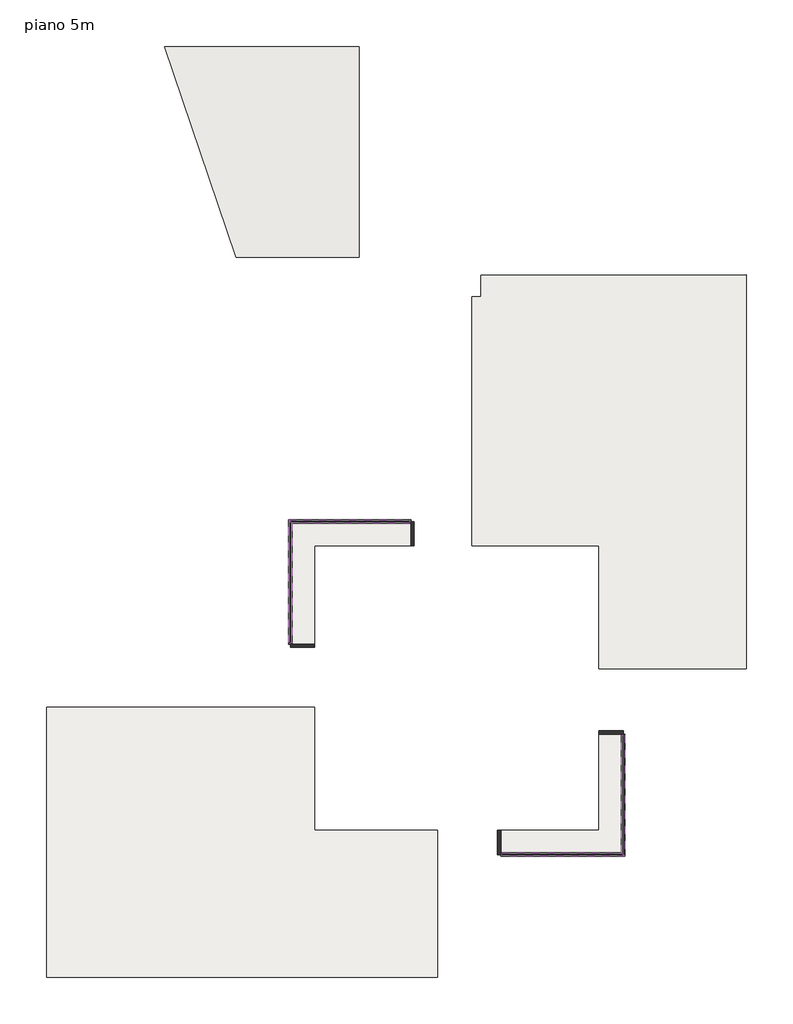
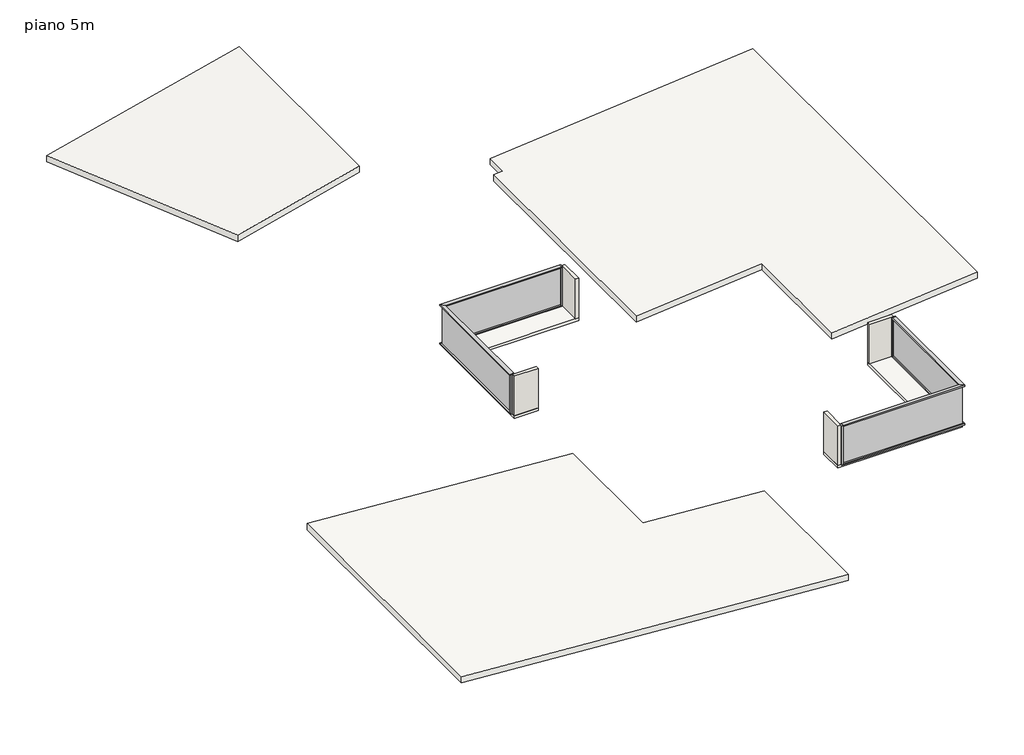
# One storey: 12 members, 4 plates, 4 walls, 3 roofs, 2 slabs.
"""IFC4 building model written with IfcOpenShell, lengths in millimetres."""

import ifcopenshell
import ifcopenshell.guid

model = None  # the IFC model being written
_history = None  # IfcOwnerHistory: only IFC2X3 demands one
_inside = {}  # id of a spatial element -> (the spatial element, [elements in it])
_under = {}  # id of a project, library or spatial element -> (it, [spatial elements below it])
_declared = {}  # id of a project -> (the project, [libraries it declares])
_typed = {}  # id of a type object -> (the type object, [elements of that type])
_made_of = {}  # id of a material, layer set ... -> (it, [elements and type objects made of it])


def new_model(schema):
    """Start an empty IFC model of exactly this schema.

    Asked for "IFC4X3", IfcOpenShell would pick the latest addendum, in which some entities
    have other attributes; the version numbers below select the first issue.
    IFC2X3 requires an IfcOwnerHistory on every rooted entity: one is made here for all.
    """
    global model, _history
    if schema == "IFC4X3":
        model = ifcopenshell.file(schema_version=(4, 3, 0, 0))
    else:
        model = ifcopenshell.file(schema=schema)
    _inside.clear()
    _under.clear()
    _declared.clear()
    _typed.clear()
    _made_of.clear()
    _history = None
    if model.schema == "IFC2X3":
        org = make("IfcOrganization", Name="unknown")
        user = make(
            "IfcPersonAndOrganization",
            ThePerson=make("IfcPerson", FamilyName="unknown"),
            TheOrganization=org,
        )
        app = make(
            "IfcApplication",
            ApplicationDeveloper=org,
            Version="unknown",
            ApplicationFullName="unknown",
            ApplicationIdentifier="unknown",
        )
        _history = make(
            "IfcOwnerHistory",
            OwningUser=user,
            OwningApplication=app,
            ChangeAction="ADDED",
            CreationDate=0,
        )
    return model


def make(cls, **values):
    """One entity of the class cls with the attributes given. An attribute that is None is left unset."""
    return model.create_entity(
        cls, **{name: value for name, value in values.items() if value is not None}
    )


def rooted(cls, **values):
    """An entity with a GlobalId (a new one), such as an element, a storey or a relation."""
    return make(cls, GlobalId=ifcopenshell.guid.new(), OwnerHistory=_history, **values)


def si_unit(unit_type, name, prefix=None):
    """IfcSIUnit, for example si_unit("LENGTHUNIT", "METRE", prefix="MILLI")."""
    return make("IfcSIUnit", UnitType=unit_type, Prefix=prefix, Name=name)


def assignment(units):
    """IfcUnitAssignment: the units of a project."""
    return None if units is None else make("IfcUnitAssignment", Units=units)


def point(xyz):
    """IfcCartesianPoint."""
    return None if xyz is None else make("IfcCartesianPoint", Coordinates=xyz)


def direction(xyz):
    """IfcDirection."""
    return None if xyz is None else make("IfcDirection", DirectionRatios=xyz)


def frame(location, z_axis=None, x_axis=None):
    """IfcAxis2Placement3D, a coordinate frame: its origin and axes. An axis left out is left unset."""
    return make(
        "IfcAxis2Placement3D",
        Location=point(location),
        Axis=direction(z_axis),
        RefDirection=direction(x_axis),
    )


def origin():
    """The frame at (0, 0, 0) with its axes left unset."""
    return frame((0.0, 0.0, 0.0))


def origin_with_axes():
    """The frame at (0, 0, 0) with the z axis (0, 0, 1) and the x axis (1, 0, 0) written out."""
    return frame((0.0, 0.0, 0.0), z_axis=(0.0, 0.0, 1.0), x_axis=(1.0, 0.0, 0.0))


def place(relative_to, where):
    """IfcLocalPlacement: puts the frame where relative to a parent placement (None: the world)."""
    return make(
        "IfcLocalPlacement", PlacementRelTo=relative_to, RelativePlacement=where
    )


def context(
    kind, dimensions, precision=None, world=None, true_north=None, identifier=None
):
    """IfcGeometricRepresentationContext, for example the 3D "Model" context."""
    return make(
        "IfcGeometricRepresentationContext",
        ContextIdentifier=identifier,
        ContextType=kind,
        CoordinateSpaceDimension=dimensions,
        Precision=precision,
        WorldCoordinateSystem=world,
        TrueNorth=true_north,
    )


def project(units=None, contexts=None):
    """IfcProject with its units and contexts."""
    return rooted(
        "IfcProject",
        Name="project",
        RepresentationContexts=contexts,
        UnitsInContext=assignment(units),
    )


def spatial(cls, under=None, at=None, **own):
    """A site, building, storey or space (cls), placed at a placement, below another one or the project."""
    s = rooted(cls, ObjectPlacement=at, **own)
    if under is not None:
        _under.setdefault(under.id(), (under, []))[1].append(s)
    return s


def polyline(points):
    """IfcPolyline through the points."""
    return make("IfcPolyline", Points=[point(p) for p in points])


def outline(outer, holes=None, kind="AREA"):
    """IfcArbitraryClosedProfileDef: a profile drawn as a closed curve; with holes, ...WithVoids."""
    if holes is None:
        return make("IfcArbitraryClosedProfileDef", ProfileType=kind, OuterCurve=outer)
    return make(
        "IfcArbitraryProfileDefWithVoids",
        ProfileType=kind,
        OuterCurve=outer,
        InnerCurves=holes,
    )


def extrude(swept, where, along, depth):
    """IfcExtrudedAreaSolid: the profile swept, set in the frame where, extruded along a direction by depth."""
    return make(
        "IfcExtrudedAreaSolid",
        SweptArea=swept,
        Position=where,
        ExtrudedDirection=direction(along),
        Depth=depth,
    )


def faces_of(points, faces, orient=None, outer=None):
    """IfcFace entities. A face is a list of loops; a loop is a list of indices into points, from 0.

    orient and outer hold one flag for each loop. By default every Orientation is true, the
    first loop of a face is its IfcFaceOuterBound and the others are IfcFaceBound.
    """
    made = []
    for i, loops in enumerate(faces):
        bounds = []
        for j, loop in enumerate(loops):
            is_outer = j == 0 if outer is None else outer[i][j]
            bounds.append(
                make(
                    "IfcFaceOuterBound" if is_outer else "IfcFaceBound",
                    Bound=make("IfcPolyLoop", Polygon=[points[k] for k in loop]),
                    Orientation=True if orient is None else orient[i][j],
                )
            )
        made.append(make("IfcFace", Bounds=bounds))
    return made


def faceted_brep(points, faces, orient=None, outer=None, voids=None):
    """IfcFacetedBrep: a solid bounded by flat faces; with voids (closed shells), ...WithVoids."""
    shared = [point(p) for p in points]
    hull = make("IfcClosedShell", CfsFaces=faces_of(shared, faces, orient, outer))
    if voids is None:
        return make("IfcFacetedBrep", Outer=hull)
    return make(
        "IfcFacetedBrepWithVoids",
        Outer=hull,
        Voids=[
            make(cls, CfsFaces=faces_of(shared, fs, o, b)) for cls, fs, o, b in voids
        ],
    )


def shape(context_of_items, identifier, shape_type, items):
    """IfcShapeRepresentation: the items that make up one representation, for example the "Body"."""
    return make(
        "IfcShapeRepresentation",
        ContextOfItems=context_of_items,
        RepresentationIdentifier=identifier,
        RepresentationType=shape_type,
        Items=items,
    )


def source(mapping_origin, context_of_items, identifier, shape_type, items):
    """IfcRepresentationMap: a shape defined once, which mapped items show again and again."""
    return make(
        "IfcRepresentationMap",
        MappingOrigin=mapping_origin,
        MappedRepresentation=shape(context_of_items, identifier, shape_type, items),
    )


def transform(
    local_origin,
    x_axis=None,
    y_axis=None,
    z_axis=None,
    scale=None,
    scale2=None,
    scale3=None,
    uniform=True,
):
    """IfcCartesianTransformationOperator3D, or its non-uniform kind. x_axis, y_axis, z_axis: its Axis1, 2, 3."""
    if uniform:
        return make(
            "IfcCartesianTransformationOperator3D",
            Axis1=direction(x_axis),
            Axis2=direction(y_axis),
            LocalOrigin=point(local_origin),
            Scale=scale,
            Axis3=direction(z_axis),
        )
    return make(
        "IfcCartesianTransformationOperator3DnonUniform",
        Axis1=direction(x_axis),
        Axis2=direction(y_axis),
        LocalOrigin=point(local_origin),
        Scale=scale,
        Axis3=direction(z_axis),
        Scale2=scale2,
        Scale3=scale3,
    )


def mapped(mapping_source, mapping_target):
    """IfcMappedItem: shows the shape of a source again, moved by a transform."""
    return make(
        "IfcMappedItem", MappingSource=mapping_source, MappingTarget=mapping_target
    )


def made_of(thing, what):
    """Note that an element or type object is made of a material, layer set ...; save() writes the relation."""
    if what is not None:
        _made_of.setdefault(what.id(), (what, []))[1].append(thing)
    return thing


def element(
    cls,
    number,
    at=None,
    inside=None,
    cuts=None,
    type_object=None,
    material=None,
    context=None,
    identifier="Body",
    shape_type=None,
    held_by="IfcProductDefinitionShape",
    body=None,
    shapes=None,
    **own,
):
    """One element of the class cls, such as IfcWall. Its Tag is "e" and its number.

    at: its placement. inside: the storey or other place that contains it. cuts: it is an
    opening in that element (IfcRelVoidsElement). A single representation is given by context,
    identifier, shape_type and body (its items); several are given by shapes. held_by: the class
    of the entity that holds the representations. save() writes the other relations.
    """
    e = rooted(cls, Tag="e%d" % number, ObjectPlacement=at, **own)
    if body is not None:
        shapes = [shape(context, identifier, shape_type, body)]
    if shapes is not None:
        e.Representation = make(held_by, Representations=shapes)
    if inside is not None:
        _inside.setdefault(inside.id(), (inside, []))[1].append(e)
    if cuts is not None:
        rooted(
            "IfcRelVoidsElement", RelatingBuildingElement=cuts, RelatedOpeningElement=e
        )
    if type_object is not None:
        _typed.setdefault(type_object.id(), (type_object, []))[1].append(e)
    return made_of(e, material)


def aggregate(whole, parts):
    """IfcRelAggregates: a whole, such as a stair, and the parts it consists of."""
    return rooted("IfcRelAggregates", RelatingObject=whole, RelatedObjects=parts)


def save(model, path):
    """Write the relations noted so far, then the file.

    IfcRelAggregates (storeys below a building ...), IfcRelContainedInSpatialStructure (elements
    in a storey), IfcRelDefinesByType, IfcRelAssociatesMaterial and IfcRelDeclares: one each for
    every whole, place, type object, material and project.
    """
    for whole, parts in _under.values():
        aggregate(whole, parts)
    for where, things in _inside.values():
        rooted(
            "IfcRelContainedInSpatialStructure",
            RelatedElements=things,
            RelatingStructure=where,
        )
    for kind, things in _typed.values():
        rooted("IfcRelDefinesByType", RelatedObjects=things, RelatingType=kind)
    for what, things in _made_of.values():
        rooted("IfcRelAssociatesMaterial", RelatedObjects=things, RelatingMaterial=what)
    for by, libraries in _declared.values():
        rooted("IfcRelDeclares", RelatingContext=by, RelatedDefinitions=libraries)
    model.write(path)


def montante_rettangolare_montante_rettangolare_b878ced1(model_context):
    return source(origin(), model_context, "Body", "SweptSolid", [
        extrude(outline(polyline([(0.0, 75.0), (0.0, -75.0), (-50.0, -75.0), (-50.0, 75.0), (0.0, 75.0)])), frame((0.0, 0.0, -1745.0), z_axis=(0.0, 0.0, 1.0), x_axis=(1.0, 0.0, 0.0)), (0.0, 0.0, 1.0), 1745.0),
    ])


def montante_rettangolare_montante_rettangolare_f37d3d93(model_context):
    return source(origin(), model_context, "Body", "SweptSolid", [
        extrude(outline(polyline([(-75.0, -75.0), (75.0, 75.0), (75.0, -4920.0), (-75.0, -4920.0), (-75.0, -75.0)])), frame((-50.0, 0.0, 0.0), z_axis=(1.0, 0.0, 0.0), x_axis=(0.0, 1.0, 0.0)), (0.0, 0.0, 1.0), 50.0),
    ])


def montante_rettangolare_montante_rettangolare_ca0860d7(model_context):
    return source(origin(), model_context, "Body", "SweptSolid", [
        extrude(outline(polyline([(-75.0, 0.0), (75.0, 0.0), (75.0, -5080.0), (-75.0, -4930.0), (-75.0, 0.0)])), frame((-50.0, 0.0, 0.0), z_axis=(1.0, 0.0, 0.0), x_axis=(0.0, 1.0, 0.0)), (0.0, 0.0, 1.0), 50.0),
    ])


def montante_rettangolare_montante_rettangolare_c5eda454(model_context):
    return source(origin(), model_context, "Body", "SweptSolid", [
        extrude(outline(polyline([(-75.0, 0.0), (75.0, 0.0), (75.0, -4995.0), (-75.0, -4845.0), (-75.0, 0.0)])), frame((-50.0, 0.0, 0.0), z_axis=(1.0, 0.0, 0.0), x_axis=(0.0, 1.0, 0.0)), (0.0, 0.0, 1.0), 50.0),
    ])


def montante_rettangolare_montante_rettangolare_44b40ab6(model_context):
    return source(origin(), model_context, "Body", "SweptSolid", [
        extrude(outline(polyline([(-75.0, -75.0), (75.0, 75.0), (75.0, -5005.0), (-75.0, -5005.0), (-75.0, -75.0)])), frame((-50.0, 0.0, 0.0), z_axis=(1.0, 0.0, 0.0), x_axis=(0.0, 1.0, 0.0)), (0.0, 0.0, 1.0), 50.0),
    ])


def montante_rettangolare_montante_rettangolare_370ce85d(model_context):
    return source(origin(), model_context, "Body", "SweptSolid", [
        extrude(outline(polyline([(-75.0, 0.0), (75.0, 0.0), (75.0, -4845.0), (-75.0, -4995.0), (-75.0, 0.0)])), frame((-50.0, 0.0, 0.0), z_axis=(1.0, 0.0, 0.0), x_axis=(0.0, 1.0, 0.0)), (0.0, 0.0, 1.0), 50.0),
    ])


def montante_rettangolare_montante_rettangolare_df59e700(model_context):
    return source(origin(), model_context, "Body", "SweptSolid", [
        extrude(outline(polyline([(-75.0, 75.0), (75.0, -75.0), (75.0, -5005.0), (-75.0, -5005.0), (-75.0, 75.0)])), frame((-50.0, 0.0, 0.0), z_axis=(1.0, 0.0, 0.0), x_axis=(0.0, 1.0, 0.0)), (0.0, 0.0, 1.0), 50.0),
    ])


def montante_rettangolare_montante_rettangolare_9078f481(model_context):
    return source(origin(), model_context, "Body", "SweptSolid", [
        extrude(outline(polyline([(-75.0, 0.0), (75.0, 0.0), (75.0, -4930.0), (-75.0, -5080.0), (-75.0, 0.0)])), frame((-50.0, 0.0, 0.0), z_axis=(1.0, 0.0, 0.0), x_axis=(0.0, 1.0, 0.0)), (0.0, 0.0, 1.0), 50.0),
    ])


def montante_rettangolare_montante_rettangolare_efcb39a4(model_context):
    return source(origin(), model_context, "Body", "SweptSolid", [
        extrude(outline(polyline([(-75.0, 75.0), (75.0, -75.0), (75.0, -4920.0), (-75.0, -4920.0), (-75.0, 75.0)])), frame((-50.0, 0.0, 0.0), z_axis=(1.0, 0.0, 0.0), x_axis=(0.0, 1.0, 0.0)), (0.0, 0.0, 1.0), 50.0),
    ])


def pannello_sistema_vetrato_c31b63d1(model_context):
    return source(origin(), model_context, "Body", "SweptSolid", [
        extrude(outline(polyline([(2502.5, -15.0), (-2502.5, -15.0), (-2502.5, 15.0), (2502.5, 15.0), (2502.5, -15.0)])), origin_with_axes(), (0.0, 0.0, 1.0), 1645.0),
    ])


def pannello_sistema_vetrato_f11d9790(model_context):
    return source(origin(), model_context, "Body", "SweptSolid", [
        extrude(outline(polyline([(2460.0, -15.0), (-2460.0, -15.0), (-2460.0, 15.0), (2460.0, 15.0), (2460.0, -15.0)])), origin_with_axes(), (0.0, 0.0, 1.0), 1645.0),
    ])


model = new_model("IFC4")

# Units and contexts
model_context = context("Model", 3, world=origin())
ifc_project = project(units=[si_unit("LENGTHUNIT", "METRE", prefix="MILLI")], contexts=[model_context])

# Site, building, storey
site = spatial("IfcSite", under=ifc_project)
building = spatial("IfcBuilding", under=site)
storey = spatial("IfcBuildingStorey", under=building, Name="piano 5m", Elevation=5000.0)

# Members
placement = place(None, origin())
montante_rettangolare_montante_rettangolare_shape = montante_rettangolare_montante_rettangolare_b878ced1(model_context)
element("IfcMember", 1, ObjectType="Montante rettangolare : Montante rettangolare", at=placement, inside=storey, context=model_context, shape_type="MappedRepresentation", body=[
    mapped(montante_rettangolare_montante_rettangolare_shape, transform((-2934.088537, 278.6009057, 6745.0), x_axis=(1.0, 0.0, 0.0), y_axis=(0.0, 1.0, 0.0), z_axis=(0.0, 0.0, 1.0))),
])
element("IfcMember", 2, ObjectType="Montante rettangolare : Montante rettangolare", at=placement, inside=storey, context=model_context, shape_type="MappedRepresentation", body=[
    mapped(montante_rettangolare_montante_rettangolare_shape, transform((-7904.088537, -4776.3990943, 5000.0), x_axis=(0.0, -1.0, 0.0), y_axis=(-1.0, 0.0, 0.0), z_axis=(0.0, 0.0, -1.0))),
])
montante_rettangolare_montante_rettangolare_2_shape = montante_rettangolare_montante_rettangolare_f37d3d93(model_context)
element("IfcMember", 3, ObjectType="Montante rettangolare : Montante rettangolare", at=placement, inside=storey, context=model_context, shape_type="MappedRepresentation", body=[
    mapped(montante_rettangolare_montante_rettangolare_2_shape, transform((-7904.088537, 278.6009057, 6745.0), x_axis=(0.0, 0.0, 1.0), y_axis=(0.0, 1.0, 0.0), z_axis=(-1.0, 0.0, 0.0))),
])
montante_rettangolare_montante_rettangolare_3_shape = montante_rettangolare_montante_rettangolare_ca0860d7(model_context)
element("IfcMember", 4, ObjectType="Montante rettangolare : Montante rettangolare", at=placement, inside=storey, context=model_context, shape_type="MappedRepresentation", body=[
    mapped(montante_rettangolare_montante_rettangolare_3_shape, transform((-7904.088537, -4726.3990943, 6745.0), x_axis=(0.0, 0.0, 1.0), y_axis=(-1.0, 0.0, 0.0), z_axis=(0.0, -1.0, 0.0))),
])
montante_rettangolare_montante_rettangolare_4_shape = montante_rettangolare_montante_rettangolare_c5eda454(model_context)
element("IfcMember", 5, ObjectType="Montante rettangolare : Montante rettangolare", at=placement, inside=storey, context=model_context, shape_type="MappedRepresentation", body=[
    mapped(montante_rettangolare_montante_rettangolare_4_shape, transform((-2984.088537, 278.6009057, 5000.0), x_axis=(0.0, 0.0, -1.0), y_axis=(0.0, 1.0, 0.0), z_axis=(1.0, 0.0, 0.0))),
])
montante_rettangolare_montante_rettangolare_5_shape = montante_rettangolare_montante_rettangolare_44b40ab6(model_context)
element("IfcMember", 6, ObjectType="Montante rettangolare : Montante rettangolare", at=placement, inside=storey, context=model_context, shape_type="MappedRepresentation", body=[
    mapped(montante_rettangolare_montante_rettangolare_5_shape, transform((-7904.088537, 278.6009057, 5000.0), x_axis=(0.0, 0.0, -1.0), y_axis=(-1.0, 0.0, 0.0), z_axis=(0.0, 1.0, 0.0))),
])
montante_rettangolare_montante_rettangolare_6_shape = montante_rettangolare_montante_rettangolare_370ce85d(model_context)
element("IfcMember", 7, ObjectType="Montante rettangolare : Montante rettangolare", at=placement, inside=storey, context=model_context, shape_type="MappedRepresentation", body=[
    mapped(montante_rettangolare_montante_rettangolare_6_shape, transform((5835.911463, -8541.3990943, 5000.0), x_axis=(0.0, 0.0, -1.0), y_axis=(-1.0, 0.0, 0.0), z_axis=(0.0, 1.0, 0.0))),
])
montante_rettangolare_montante_rettangolare_7_shape = montante_rettangolare_montante_rettangolare_df59e700(model_context)
element("IfcMember", 8, ObjectType="Montante rettangolare : Montante rettangolare", at=placement, inside=storey, context=model_context, shape_type="MappedRepresentation", body=[
    mapped(montante_rettangolare_montante_rettangolare_7_shape, transform((5835.911463, -13461.3990943, 5000.0), x_axis=(0.0, 0.0, -1.0), y_axis=(0.0, 1.0, 0.0), z_axis=(1.0, 0.0, 0.0))),
])
element("IfcMember", 9, ObjectType="Montante rettangolare : Montante rettangolare", at=placement, inside=storey, context=model_context, shape_type="MappedRepresentation", body=[
    mapped(montante_rettangolare_montante_rettangolare_shape, transform((5835.911463, -8491.3990943, 6745.0), x_axis=(0.0, 1.0, 0.0), y_axis=(-1.0, 0.0, 0.0), z_axis=(0.0, 0.0, 1.0))),
])
element("IfcMember", 10, ObjectType="Montante rettangolare : Montante rettangolare", at=placement, inside=storey, context=model_context, shape_type="MappedRepresentation", body=[
    mapped(montante_rettangolare_montante_rettangolare_shape, transform((780.911463, -13461.3990943, 5000.0), x_axis=(-1.0, 0.0, 0.0), y_axis=(0.0, 1.0, 0.0), z_axis=(0.0, 0.0, -1.0))),
])
montante_rettangolare_montante_rettangolare_8_shape = montante_rettangolare_montante_rettangolare_9078f481(model_context)
element("IfcMember", 11, ObjectType="Montante rettangolare : Montante rettangolare", at=placement, inside=storey, context=model_context, shape_type="MappedRepresentation", body=[
    mapped(montante_rettangolare_montante_rettangolare_8_shape, transform((830.911463, -13461.3990943, 6745.0), x_axis=(0.0, 0.0, 1.0), y_axis=(0.0, 1.0, 0.0), z_axis=(-1.0, 0.0, 0.0))),
])
montante_rettangolare_montante_rettangolare_9_shape = montante_rettangolare_montante_rettangolare_efcb39a4(model_context)
element("IfcMember", 12, ObjectType="Montante rettangolare : Montante rettangolare", at=placement, inside=storey, context=model_context, shape_type="MappedRepresentation", body=[
    mapped(montante_rettangolare_montante_rettangolare_9_shape, transform((5835.911463, -13461.3990943, 6745.0), x_axis=(0.0, 0.0, 1.0), y_axis=(-1.0, 0.0, 0.0), z_axis=(0.0, -1.0, 0.0))),
])

# Plates
pannello_sistema_vetrato_shape = pannello_sistema_vetrato_c31b63d1(model_context)
element("IfcPlate", 13, ObjectType="Pannello sistema : Vetrato", at=placement, inside=storey, context=model_context, shape_type="MappedRepresentation", body=[
    mapped(pannello_sistema_vetrato_shape, transform((-7904.088537, -2223.8990943, 5050.0), x_axis=(0.0, -1.0, 0.0), y_axis=(1.0, 0.0, 0.0), z_axis=(0.0, 0.0, 1.0))),
])
pannello_sistema_vetrato_2_shape = pannello_sistema_vetrato_f11d9790(model_context)
element("IfcPlate", 14, ObjectType="Pannello sistema : Vetrato", at=placement, inside=storey, context=model_context, shape_type="MappedRepresentation", body=[
    mapped(pannello_sistema_vetrato_2_shape, transform((-5444.088537, 278.6009057, 5050.0), x_axis=(-1.0, 0.0, 0.0), y_axis=(0.0, -1.0, 0.0), z_axis=(0.0, 0.0, 1.0))),
])
element("IfcPlate", 15, ObjectType="Pannello sistema : Vetrato", at=placement, inside=storey, context=model_context, shape_type="MappedRepresentation", body=[
    mapped(pannello_sistema_vetrato_2_shape, transform((5835.911463, -11001.3990943, 5050.0), x_axis=(0.0, -1.0, 0.0), y_axis=(1.0, 0.0, 0.0), z_axis=(0.0, 0.0, 1.0))),
])
element("IfcPlate", 16, ObjectType="Pannello sistema : Vetrato", at=placement, inside=storey, context=model_context, shape_type="MappedRepresentation", body=[
    mapped(pannello_sistema_vetrato_shape, transform((3333.411463, -13461.3990943, 5050.0), x_axis=(-1.0, 0.0, 0.0), y_axis=(0.0, -1.0, 0.0), z_axis=(0.0, 0.0, 1.0))),
])

# Roofs
element("IfcRoof", 17, ObjectType="Latero Cementizio - 27 cm", at=placement, inside=storey, context=model_context, shape_type="Brep", body=[
    faceted_brep([(-17974.088537, -7391.3990943, 5270.6593125), (-6904.088537, -7391.3990943, 4496.5695043), (-6904.088537, -7391.3990943, 4225.9101918), (-17974.088537, -7391.3990943, 5000.0), (-1834.088537, -12461.3990943, 4142.0405677), (-1834.088537, -18531.3990943, 4142.0405677), (-1834.088537, -18531.3990943, 3871.3812552), (-1834.088537, -12461.3990943, 3871.3812552), (-6904.088537, -12461.3990943, 4496.5695043), (-6904.088537, -12461.3990943, 4225.9101918), (-17974.088537, -18531.3990943, 5000.0), (-17974.088537, -18531.3990943, 5270.6593125)], [[[0, 1, 2, 3]], [[4, 5, 6, 7]], [[1, 8, 9, 2]], [[8, 4, 7, 9]], [[6, 10, 3, 2, 9, 7]], [[11, 5, 4, 8, 1, 0]], [[10, 11, 0, 3]], [[5, 11, 10, 6]]]),
])
element("IfcRoof", 18, ObjectType="Latero Cementizio - 27 cm", at=placement, inside=storey, context=model_context, shape_type="Brep", body=[
    faceted_brep([(10905.911463, -5791.3990943, 5018.553439), (4835.911463, -5791.3990943, 4455.4565641), (4835.911463, -721.3990943, 4455.4565641), (-404.088537, -721.3990943, 3969.3564613), (-404.088537, 9548.6009057, 3969.3564613), (-34.088537, 9548.6009057, 4003.6803235), (-34.088537, 10448.6009057, 4003.6803235), (10905.911463, 10448.6009057, 5018.553439), (4835.911463, -5791.3990943, 4726.6158519), (10905.911463, -5791.3990943, 5289.7127268), (10905.911463, 10448.6009057, 5289.7127268), (-34.088537, 10448.6009057, 4274.8396113), (-34.088537, 9548.6009057, 4274.8396113), (-404.088537, 9548.6009057, 4240.5157491), (-404.088537, -721.3990943, 4240.5157491), (4835.911463, -721.3990943, 4726.6158519)], [[[0, 1, 2, 3, 4, 5, 6, 7]], [[8, 9, 10, 11, 12, 13, 14, 15]], [[7, 10, 9, 0]], [[9, 8, 1, 0]], [[11, 10, 7, 6]], [[15, 14, 3, 2]], [[8, 15, 2, 1]], [[14, 13, 4, 3]], [[13, 12, 5, 4]], [[12, 11, 6, 5]]]),
])
element("IfcRoof", 19, ObjectType="Latero Cementizio - 27 cm", at=placement, inside=storey, context=model_context, shape_type="Brep", body=[
    faceted_brep([(-13107.7585057, 19873.6009057, 2998.1110261), (-5078.6203781, 19873.6009057, 5000.0), (-5078.6203781, 11173.6009057, 5000.0), (-10157.5612554, 11173.6009057, 3733.6778145), (-5078.6203781, 19873.6009057, 5278.2656799), (-13107.7585057, 19873.6009057, 3276.376706), (-10157.5612554, 11173.6009057, 4011.9434944), (-5078.6203781, 11173.6009057, 5278.2656799)], [[[0, 1, 2, 3]], [[4, 5, 6, 7]], [[1, 4, 7, 2]], [[5, 4, 1, 0]], [[6, 5, 0, 3]], [[7, 6, 3, 2]]]),
])

# Slabs
element("IfcSlab", 20, ObjectType="per finestre 12cm", at=placement, inside=storey, context=model_context, shape_type="SweptSolid", body=[
    extrude(outline(polyline([(4835.911463, -12461.3990943), (4835.911463, -8361.3990943), (5835.911463, -8361.3990943), (5835.911463, -13461.3990943), (650.911463, -13461.3990943), (650.911463, -12461.3990943), (4835.911463, -12461.3990943)])), frame((0.0, 0.0, 4880.0), z_axis=(0.0, 0.0, 1.0), x_axis=(1.0, 0.0, 0.0)), (0.0, 0.0, 1.0), 120.0),
])
element("IfcSlab", 21, ObjectType="per finestre 12cm", at=placement, inside=storey, context=model_context, shape_type="SweptSolid", body=[
    extrude(outline(polyline([(-6904.088537, -721.3990943), (-6904.088537, -4906.3990943), (-7904.088537, -4906.3990943), (-7904.088537, 278.6009057), (-2804.088537, 278.6009057), (-2804.088537, -721.3990943), (-6904.088537, -721.3990943)])), frame((0.0, 0.0, 4880.0), z_axis=(0.0, 0.0, 1.0), x_axis=(1.0, 0.0, 0.0)), (0.0, 0.0, 1.0), 120.0),
])

# Walls
element("IfcWall", 22, ObjectType="tramezzo 12cm", at=placement, inside=storey, context=model_context, shape_type="SweptSolid", body=[
    extrude(outline(polyline([(780.911463, -12461.3990943), (780.911463, -13461.3990943), (650.911463, -13461.3990943), (650.911463, -12461.3990943), (780.911463, -12461.3990943)])), frame((0.0, 0.0, 5000.0), z_axis=(0.0, 0.0, 1.0), x_axis=(1.0, 0.0, 0.0)), (0.0, 0.0, 1.0), 1745.0),
])
element("IfcWall", 23, ObjectType="tramezzo 12cm", at=placement, inside=storey, context=model_context, shape_type="SweptSolid", body=[
    extrude(outline(polyline([(4835.911463, -8361.3990943), (5835.911463, -8361.3990943), (5835.911463, -8491.3990943), (4835.911463, -8491.3990943), (4835.911463, -8361.3990943)])), frame((0.0, 0.0, 5000.0), z_axis=(0.0, 0.0, 1.0), x_axis=(1.0, 0.0, 0.0)), (0.0, 0.0, 1.0), 1745.0),
])
element("IfcWall", 24, ObjectType="tramezzo 12cm", at=placement, inside=storey, context=model_context, shape_type="SweptSolid", body=[
    extrude(outline(polyline([(-6904.088537, -4906.3990943), (-7904.088537, -4906.3990943), (-7904.088537, -4776.3990943), (-6904.088537, -4776.3990943), (-6904.088537, -4906.3990943)])), frame((0.0, 0.0, 5000.0), z_axis=(0.0, 0.0, 1.0), x_axis=(1.0, 0.0, 0.0)), (0.0, 0.0, 1.0), 1745.0),
])
element("IfcWall", 25, ObjectType="tramezzo 12cm", at=placement, inside=storey, context=model_context, shape_type="SweptSolid", body=[
    extrude(outline(polyline([(-2934.088537, -721.3990943), (-2934.088537, 278.6009057), (-2804.088537, 278.6009057), (-2804.088537, -721.3990943), (-2934.088537, -721.3990943)])), frame((0.0, 0.0, 5000.0), z_axis=(0.0, 0.0, 1.0), x_axis=(1.0, 0.0, 0.0)), (0.0, 0.0, 1.0), 1745.0),
])

save(model, "model.ifc")

# Revit data of these elements
# Project information
#   Data di consegna del progetto = "Data"
#   Stato del progetto = "Stato"
#   Nome del cliente = "Proprietario"
#   Nome del progetto = "Nome"
#   Numero del progetto = "0001"
# Type "Montante rettangolare : Montante rettangolare"
#   built-in parameter 1007304 = 0.492126 (stored number, unit not read)
#   built-in parameter 1007301 = 0.082021 (stored number, unit not read)
#   built-in parameter 1007300 = 0.082021 (stored number, unit not read)
# Type "Pannello sistema : Vetrato"
#   Construction Type Id = "GSP4R"
#   Analytic Construction = "Vetrata singola Pilkington 1/8 in"
#   Visual Light Transmittance = 0.9
#   Solar Heat Gain Coefficient = 0.86
#   Heat Transfer Coefficient (U) = 6.7069 W/(m²·K)
# Type "Latero Cementizio - 27 cm"
#   Keynote = "T/1"
#   Layers, outside or top first: 0.05 m "Coppi" (function 4); 0.04 m "Calcestruzzo" (function 2); 0.16 m "Laterizio (2)" (function 1); 0.02 m "Intonaco - Bianco" (function 5)
# Type "per finestre 12cm"
#   Keynote = "S/3"
#   Function = 0
#   Layers, outside or top first: 0.01 m "Ceramica bianca" (function 4); 0.02 m "Sabbia e Calcestruzzo" (function 2); 0.03 m "Calcestruzzo" (function 1); 0.05 m "Laterizio (2)" (function 1); 0.01 m "Intonaco - Bianco" (function 5)
# Type "tramezzo 12cm"
#   Keynote = "Mb/3"
#   Layers, outside or top first: 0.03 m "Intonaco - Bianco" (function 4); 0.08 m "calcestruzzo blocchi" (function 1); 0.02 m "Intonaco - Bianco" (function 5)
# Elements 1, 2, 3, 4, 5, 6, 7, 8, 9, 10, 11, 12 (IfcMember, "Montante rettangolare : Montante rettangolare")
#   Phase Created = Stato di Progetto
#   Materials on its faces: "Acciaio"
# Elements 13, 14, 15, 16 (IfcPlate, "Pannello sistema : Vetrato")
#   Phase Created = Stato di Progetto
#   Materials on its faces: "Default - Vetro"
# Element 17 (IfcRoof, "Latero Cementizio - 27 cm")
#   built-in parameter 1001705 = 17.2922 (stored number, unit not read)
#   built-in parameter 1001710 = 33615
#   Phase Created = Stato di Progetto
#   Materials on its faces: "Intonaco - Bianco", "Coppi"
# Element 18 (IfcRoof, "Latero Cementizio - 27 cm")
#   built-in parameter 1001705 = 17.3547 (stored number, unit not read)
#   built-in parameter 1001710 = 33615
#   Phase Created = Stato di Progetto
#   Materials on its faces: "Intonaco - Bianco", "Coppi"
# Element 19 (IfcRoof, "Latero Cementizio - 27 cm")
#   built-in parameter 1001705 = 17.3171 (stored number, unit not read)
#   built-in parameter 1001710 = 33615
#   Phase Created = Stato di Progetto
#   Materials on its faces: "Intonaco - Bianco", "Coppi"
# Element 20 (IfcSlab, "per finestre 12cm")
#   built-in parameter 1001955 = -1.5708 (stored number, unit not read)
#   Height Offset From Level = 0.00 m
#   Phase Created = Stato di Progetto
#   Materials on its faces: "Intonaco - Bianco", "Ceramica bianca"
# Element 21 (IfcSlab, "per finestre 12cm")
#   built-in parameter 1001955 = 3.14159 (stored number, unit not read)
#   Height Offset From Level = 0.00 m
#   Phase Created = Stato di Progetto
#   Materials on its faces: "Intonaco - Bianco", "Ceramica bianca"
# Elements 22, 23, 24, 25 (IfcWall, "tramezzo 12cm")
#   Top Offset = 0.00 m
#   Base Offset = 0.00 m
#   wall height = 1.745 m
#   Phase Created = Stato di Progetto
#   Base Constraint = piano 5m
#   Top Constraint = solaio finestre uffici
#   Materials on its faces: "Default - Calcestruzzo", "Intonaco - Bianco"
# Materials
#   "Coppi": class "Varie", colour RGB 194 100 86, transparency 0, Description = "Tegole in mattone", Cost = 0
#   "Calcestruzzo": class "Calcestruzzo", colour RGB 192 192 192, transparency 0, Description = "Calcestruzzo - Cemento Portland", Cost = 0
#   "Laterizio (2)": class "Mattone", colour RGB 255 128 64, transparency 0, Description = "Pignatta h 16 cm", Cost = 0
#   "Intonaco - Bianco": class "Intonaco", colour RGB 249 249 249, transparency 0, Description = "Verniciatura", Cost = 0
#   "Ceramica bianca": class "Ceramica", colour RGB 210 210 210, transparency 0, Description = "Finitura interna - Piastrelle di ceramica incollate", Cost = 0
#   "Sabbia e Calcestruzzo": class "Calcestruzzo", colour RGB 127 127 127, transparency 0, Description = "Magrone - Sabbia e cemento", Cost = 0
#   "calcestruzzo blocchi": class "Calcestruzzo", colour RGB 255 128 0, transparency 0, Description = "Calcestruzzo", Cost = 0
#   "Acciaio": class "Metallo", colour RGB 247 247 247, transparency 0, Description = "Acciaio, finitura zigrinata", Cost = 0
#   "Default - Vetro": class "Vetro", colour RGB 208 208 208, transparency 0.7, Cost = 0
#   "Default - Calcestruzzo": class "Calcestruzzo", colour RGB 192 192 192, transparency 0, Description = "Calcestruzzo", Cost = 0
